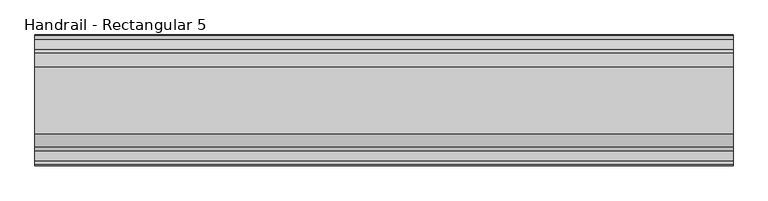
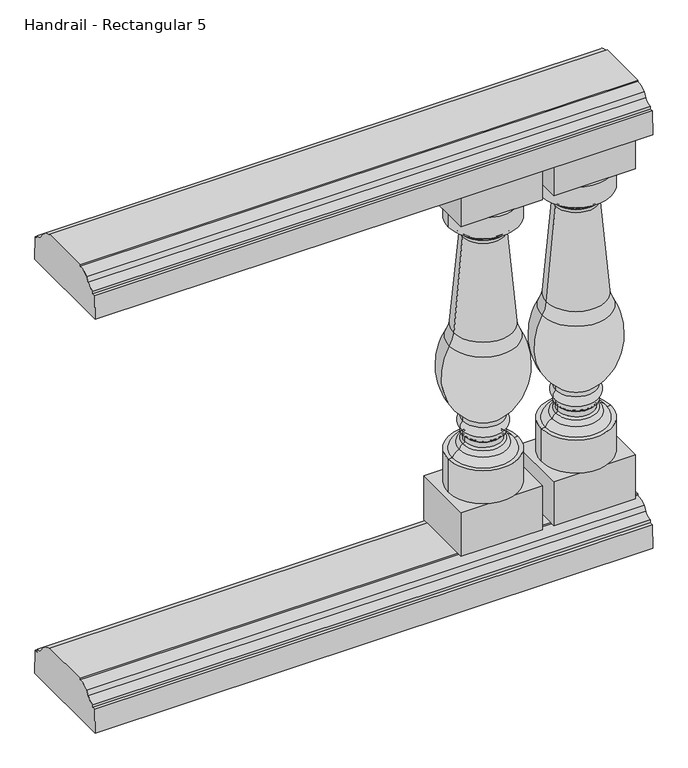
"""IFC4 building model written with IfcOpenShell, lengths in millimetres: railing geometry, Handrail - Rectangular 5."""

from ifc_helpers import new_model, si_unit, point, frame, frame_2d, origin, place, context, project, spatial, polyline, circle_curve, ellipse_curve, trimmed, segment, composite_curve, outline, extrude, source, transform, mapped, element, save
from ifc_brep_helpers import plane_surface, cylinder_surface, revolved_surface, advanced_brep


def handrail_rectangular_5_e4c3c7e0(model_context):
    return source(origin(), model_context, "Body", "SolidModel", [
        extrude(outline(composite_curve([segment(trimmed(circle_curve(frame_2d((-1771.1852268, 1054.89375)), 19.84375), [point((-1771.1852268, 1035.05))], [point((-1754.064785, 1044.8605607))], True, "CARTESIAN"), True, "CONTINUOUS"), segment(polyline([(-1754.064785, 1044.8605607), (-1747.604713, 1054.3201059)]), True, "CONTINUOUS"), segment(trimmed(circle_curve(frame_2d((-1723.5602268, 1027.90625)), 35.71875), [point((-1747.604713, 1054.3201059))], [point((-1723.5602268, 1063.625))], False, "CARTESIAN"), True, "CONTINUOUS"), segment(polyline([(-1723.5602268, 1063.625), (-1723.5602268, 1066.8), (-1607.6727268, 1066.8), (-1607.6727268, 1063.625)]), True, "CONTINUOUS"), segment(trimmed(circle_curve(frame_2d((-1607.6727268, 1027.90625)), 35.71875), [point((-1607.6727268, 1063.625))], [point((-1583.6282406, 1054.3201059))], False, "CARTESIAN"), True, "CONTINUOUS"), segment(polyline([(-1583.6282406, 1054.3201059), (-1577.1681686, 1044.8605607)]), True, "CONTINUOUS"), segment(trimmed(circle_curve(frame_2d((-1560.0477268, 1054.89375)), 19.84375), [point((-1577.1681686, 1044.8605607))], [point((-1560.0477268, 1035.05))], True, "CARTESIAN"), True, "CONTINUOUS"), segment(polyline([(-1560.0477268, 1035.05), (-1560.0477268, 1028.7), (-1552.9039768, 1028.7), (-1551.3164768, 974.725), (-1779.9164768, 974.725), (-1778.3289768, 1028.7), (-1771.1852268, 1028.7), (-1771.1852268, 1035.05)]), True, "CONTINUOUS")], self_intersect=False)), frame((16266.0521895, 0.0, 0.0), z_axis=(1.0, 0.0, 0.0), x_axis=(0.0, 1.0, 0.0)), (0.0, 0.0, 1.0), 1219.2),
        extrude(outline(composite_curve([segment(trimmed(circle_curve(frame_2d((-1771.1852268, 99.21875)), 19.84375), [point((-1771.1852268, 79.375))], [point((-1754.064785, 89.1855607))], True, "CARTESIAN"), True, "CONTINUOUS"), segment(polyline([(-1754.064785, 89.1855607), (-1747.604713, 98.6451059)]), True, "CONTINUOUS"), segment(trimmed(circle_curve(frame_2d((-1723.5602268, 72.23125)), 35.71875), [point((-1747.604713, 98.6451059))], [point((-1723.5602268, 107.95))], False, "CARTESIAN"), True, "CONTINUOUS"), segment(polyline([(-1723.5602268, 107.95), (-1723.5602268, 111.125), (-1607.6727268, 111.125), (-1607.6727268, 107.95)]), True, "CONTINUOUS"), segment(trimmed(circle_curve(frame_2d((-1607.6727268, 72.23125)), 35.71875), [point((-1607.6727268, 107.95))], [point((-1583.6282406, 98.6451059))], False, "CARTESIAN"), True, "CONTINUOUS"), segment(polyline([(-1583.6282406, 98.6451059), (-1577.1681686, 89.1855607)]), True, "CONTINUOUS"), segment(trimmed(circle_curve(frame_2d((-1560.0477268, 99.21875)), 19.84375), [point((-1577.1681686, 89.1855607))], [point((-1560.0477268, 79.375))], True, "CARTESIAN"), True, "CONTINUOUS"), segment(polyline([(-1560.0477268, 79.375), (-1560.0477268, 73.025), (-1552.9039768, 73.025), (-1551.3164768, 19.05), (-1779.9164768, 19.05), (-1778.3289768, 73.025), (-1771.1852268, 73.025), (-1771.1852268, 79.375)]), True, "CONTINUOUS")], self_intersect=False)), frame((16266.0521895, 0.0, 0.0), z_axis=(1.0, 0.0, 0.0), x_axis=(0.0, 1.0, 0.0)), (0.0, 0.0, 1.0), 1219.2),
        advanced_brep(
        [(17307.4521895, -1665.6164768, 873.125), (17459.8521895, -1665.6164768, 873.125), (17383.6521895, -1665.6164768, 873.125), (17307.4521895, -1665.6164768, 825.4490755), (17459.8521895, -1665.6164768, 825.4490755), (17317.4954208, -1665.6164768, 825.4490755), (17449.8089583, -1665.6164768, 825.4490755), (17328.9787107, -1665.6164768, 813.9657856), (17438.3256684, -1665.6164768, 813.9657856), (17328.9787107, -1665.6164768, 808.3461292), (17438.3256684, -1665.6164768, 808.3461292), (17334.6808978, -1665.6164768, 802.2016975), (17432.6234813, -1665.6164768, 802.2016975), (17338.0226936, -1665.6164768, 792.8428746), (17429.2816855, -1665.6164768, 792.8428746), (17319.2551876, -1665.6164768, 577.4758218), (17448.0491915, -1665.6164768, 577.4758218), (17310.237965, -1665.6164768, 549.5125844), (17457.0664141, -1665.6164768, 549.5125844), (17339.5087972, -1665.6164768, 376.7693301), (17427.7955818, -1665.6164768, 376.7693301), (17339.5087972, -1665.6164768, 366.4437154), (17427.7955818, -1665.6164768, 366.4437154), (17339.5087972, -1665.6164768, 343.8682651), (17427.7955818, -1665.6164768, 343.8682651), (17339.5087972, -1665.6164768, 333.5426504), (17427.7955818, -1665.6164768, 333.5426504), (17343.8192375, -1665.6164768, 329.2322102), (17423.4851416, -1665.6164768, 329.2322102), (17343.8192375, -1665.6164768, 317.4353211), (17423.4851416, -1665.6164768, 317.4353211), (17339.3214444, -1665.6164768, 313.1289544), (17427.9829347, -1665.6164768, 313.1289544), (17331.8009874, -1665.6164768, 303.0807869), (17435.5033917, -1665.6164768, 303.0807869), (17316.6523786, -1665.6164768, 288.925), (17450.6520004, -1665.6164768, 288.925), (17307.4521895, -1665.6164768, 288.925), (17459.8521895, -1665.6164768, 288.925), (17307.4521895, -1665.6164768, 212.725), (17459.8521895, -1665.6164768, 212.725), (17383.6521895, -1665.6164768, 212.725)],
        [
            (0, 1, circle_curve(frame((17383.6521895, -1665.6164768, 873.125), z_axis=(0.0, 0.0, 1.0), x_axis=(1.0, 0.0, 0.0)), 76.2)),
            (1, 2),
            (2, 0),
            (1, 0, circle_curve(frame((17383.6521895, -1665.6164768, 873.125), z_axis=(0.0, 0.0, 1.0), x_axis=(1.0, 0.0, 0.0)), 76.2)),
            (3, 4, circle_curve(frame((17383.6521895, -1665.6164768, 825.4490755), z_axis=(0.0, 0.0, 1.0), x_axis=(1.0, 0.0, 0.0)), 76.2)),
            (4, 1),
            (0, 3),
            (4, 3, circle_curve(frame((17383.6521895, -1665.6164768, 825.4490755), z_axis=(0.0, 0.0, 1.0), x_axis=(1.0, 0.0, 0.0)), 76.2)),
            (5, 6, circle_curve(frame((17383.6521895, -1665.6164768, 825.4490755), z_axis=(0.0, 0.0, 1.0), x_axis=(1.0, 0.0, 0.0)), 66.1567687)),
            (6, 4),
            (3, 5),
            (6, 5, circle_curve(frame((17383.6521895, -1665.6164768, 825.4490755), z_axis=(0.0, 0.0, 1.0), x_axis=(1.0, 0.0, 0.0)), 66.1567687)),
            (7, 8, circle_curve(frame((17383.6521895, -1665.6164768, 813.9657856), z_axis=(0.0, 0.0, 1.0), x_axis=(1.0, 0.0, 0.0)), 54.6734788)),
            (8, 6, circle_curve(frame((17438.3256684, -1665.6164768, 825.4490755), z_axis=(0.0, -1.0, 0.0), x_axis=(-1.0, 0.0, 0.0)), 11.4832899)),
            (5, 7, circle_curve(frame((17328.9787107, -1665.6164768, 825.4490755), z_axis=(0.0, -1.0, 0.0), x_axis=(1.0, 0.0, 0.0)), 11.4832899)),
            (8, 7, circle_curve(frame((17383.6521895, -1665.6164768, 813.9657856), z_axis=(0.0, 0.0, 1.0), x_axis=(1.0, 0.0, 0.0)), 54.6734788)),
            (9, 10, circle_curve(frame((17383.6521895, -1665.6164768, 808.3461292), z_axis=(0.0, 0.0, 1.0), x_axis=(1.0, 0.0, 0.0)), 54.6734788)),
            (10, 8),
            (7, 9),
            (10, 9, circle_curve(frame((17383.6521895, -1665.6164768, 808.3461292), z_axis=(0.0, 0.0, 1.0), x_axis=(1.0, 0.0, 0.0)), 54.6734788)),
            (11, 12, circle_curve(frame((17383.6521895, -1665.6164768, 802.2016975), z_axis=(0.0, 0.0, 1.0), x_axis=(1.0, 0.0, 0.0)), 48.9712918)),
            (12, 10, circle_curve(frame((17446.0345288, -1665.6164768, 795.4740105), z_axis=(0.0, 1.0, 0.0), x_axis=(-1.0, 0.0, 0.0)), 15.0039317)),
            (9, 11, circle_curve(frame((17321.2698503, -1665.6164768, 795.4740105), z_axis=(0.0, 1.0, 0.0), x_axis=(1.0, 0.0, 0.0)), 15.0039317)),
            (12, 11, circle_curve(frame((17383.6521895, -1665.6164768, 802.2016975), z_axis=(0.0, 0.0, 1.0), x_axis=(1.0, 0.0, 0.0)), 48.9712918)),
            (13, 14, circle_curve(frame((17383.6521895, -1665.6164768, 792.8428746), z_axis=(0.0, 0.0, 1.0), x_axis=(1.0, 0.0, 0.0)), 45.629496)),
            (14, 12, circle_curve(frame((17441.9595739, -1665.6164768, 793.5919719), z_axis=(0.0, 1.0, 0.0), x_axis=(-1.0, 0.0, 0.0)), 12.7)),
            (11, 13, circle_curve(frame((17325.3448052, -1665.6164768, 793.5919719), z_axis=(0.0, 1.0, 0.0), x_axis=(1.0, 0.0, 0.0)), 12.7)),
            (14, 13, circle_curve(frame((17383.6521895, -1665.6164768, 792.8428746), z_axis=(0.0, 0.0, 1.0), x_axis=(1.0, 0.0, 0.0)), 45.629496)),
            (15, 16, circle_curve(frame((17383.6521895, -1665.6164768, 577.4758218), z_axis=(0.0, 0.0, 1.0), x_axis=(1.0, 0.0, 0.0)), 64.3970019)),
            (16, 14, circle_curve(frame((21296.7232099, -1665.6164768, 1021.358044), z_axis=(0.0, 1.0, 0.0), x_axis=(-1.0, 0.0, 0.0)), 3874.1867698)),
            (13, 15, circle_curve(frame((13470.5811691, -1665.6164768, 1021.358044), z_axis=(0.0, 1.0, 0.0), x_axis=(1.0, 0.0, 0.0)), 3874.1867698)),
            (16, 15, circle_curve(frame((17383.6521895, -1665.6164768, 577.4758218), z_axis=(0.0, 0.0, 1.0), x_axis=(1.0, 0.0, 0.0)), 64.3970019)),
            (17, 18, circle_curve(frame((17383.6521895, -1665.6164768, 549.5125844), z_axis=(0.0, 0.0, 1.0), x_axis=(1.0, 0.0, 0.0)), 73.4142246)),
            (18, 16, circle_curve(frame((17522.5688441, -1665.6164768, 586.070457), z_axis=(0.0, 1.0, 0.0), x_axis=(-1.0, 0.0, 0.0)), 75.0136413)),
            (15, 17, circle_curve(frame((17244.735535, -1665.6164768, 586.070457), z_axis=(0.0, 1.0, 0.0), x_axis=(1.0, 0.0, 0.0)), 75.0136413)),
            (18, 17, circle_curve(frame((17383.6521895, -1665.6164768, 549.5125844), z_axis=(0.0, 0.0, 1.0), x_axis=(1.0, 0.0, 0.0)), 73.4142246)),
            (19, 20, circle_curve(frame((17383.6521895, -1665.6164768, 376.7693301), z_axis=(0.0, 0.0, 1.0), x_axis=(1.0, 0.0, 0.0)), 44.1433923)),
            (20, 18, circle_curve(frame((17334.9440648, -1665.6164768, 481.3542994), z_axis=(0.0, -1.0, 0.0), x_axis=(-1.0, 0.0, 0.0)), 139.8549964)),
            (17, 19, circle_curve(frame((17432.3603143, -1665.6164768, 481.3542994), z_axis=(0.0, -1.0, 0.0), x_axis=(1.0, 0.0, 0.0)), 139.8549964)),
            (20, 19, circle_curve(frame((17383.6521895, -1665.6164768, 376.7693301), z_axis=(0.0, 0.0, 1.0), x_axis=(1.0, 0.0, 0.0)), 44.1433923)),
            (21, 22, circle_curve(frame((17383.6521895, -1665.6164768, 366.4437154), z_axis=(0.0, 0.0, 1.0), x_axis=(1.0, 0.0, 0.0)), 44.1433923)),
            (22, 20),
            (19, 21),
            (22, 21, circle_curve(frame((17383.6521895, -1665.6164768, 366.4437154), z_axis=(0.0, 0.0, 1.0), x_axis=(1.0, 0.0, 0.0)), 44.1433923)),
            (23, 24, circle_curve(frame((17383.6521895, -1665.6164768, 343.8682651), z_axis=(0.0, 0.0, 1.0), x_axis=(1.0, 0.0, 0.0)), 44.1433923)),
            (24, 22, circle_curve(frame((17419.503554, -1665.6164768, 355.1559903), z_axis=(0.0, -1.0, 0.0), x_axis=(-1.0, 0.0, 0.0)), 14.0060867)),
            (21, 23, circle_curve(frame((17347.8008251, -1665.6164768, 355.1559903), z_axis=(0.0, -1.0, 0.0), x_axis=(1.0, 0.0, 0.0)), 14.0060867)),
            (24, 23, circle_curve(frame((17383.6521895, -1665.6164768, 343.8682651), z_axis=(0.0, 0.0, 1.0), x_axis=(1.0, 0.0, 0.0)), 44.1433923)),
            (25, 26, circle_curve(frame((17383.6521895, -1665.6164768, 333.5426504), z_axis=(0.0, 0.0, 1.0), x_axis=(1.0, 0.0, 0.0)), 44.1433923)),
            (26, 24),
            (23, 25),
            (26, 25, circle_curve(frame((17383.6521895, -1665.6164768, 333.5426504), z_axis=(0.0, 0.0, 1.0), x_axis=(1.0, 0.0, 0.0)), 44.1433923)),
            (27, 28, circle_curve(frame((17383.6521895, -1665.6164768, 329.2322102), z_axis=(0.0, 0.0, 1.0), x_axis=(1.0, 0.0, 0.0)), 39.8329521)),
            (28, 26, circle_curve(frame((17427.7955818, -1665.6164768, 329.2322102), z_axis=(0.0, 1.0, 0.0), x_axis=(-1.0, 0.0, 0.0)), 4.3104402)),
            (25, 27, circle_curve(frame((17339.5087972, -1665.6164768, 329.2322102), z_axis=(0.0, 1.0, 0.0), x_axis=(1.0, 0.0, 0.0)), 4.3104402)),
            (28, 27, circle_curve(frame((17383.6521895, -1665.6164768, 329.2322102), z_axis=(0.0, 0.0, 1.0), x_axis=(1.0, 0.0, 0.0)), 39.8329521)),
            (29, 30, circle_curve(frame((17383.6521895, -1665.6164768, 317.4353211), z_axis=(0.0, 0.0, 1.0), x_axis=(1.0, 0.0, 0.0)), 39.8329521)),
            (30, 28),
            (27, 29),
            (30, 29, circle_curve(frame((17383.6521895, -1665.6164768, 317.4353211), z_axis=(0.0, 0.0, 1.0), x_axis=(1.0, 0.0, 0.0)), 39.8329521)),
            (31, 32, circle_curve(frame((17383.6521895, -1665.6164768, 313.1289544), z_axis=(0.0, 0.0, 1.0), x_axis=(1.0, 0.0, 0.0)), 44.3307451)),
            (32, 30, circle_curve(frame((17427.7955818, -1665.6164768, 317.4353211), z_axis=(0.0, 1.0, 0.0), x_axis=(-1.0, 0.0, 0.0)), 4.3104402)),
            (29, 31, circle_curve(frame((17339.5087972, -1665.6164768, 317.4353211), z_axis=(0.0, 1.0, 0.0), x_axis=(1.0, 0.0, 0.0)), 4.3104402)),
            (32, 31, circle_curve(frame((17383.6521895, -1665.6164768, 313.1289544), z_axis=(0.0, 0.0, 1.0), x_axis=(1.0, 0.0, 0.0)), 44.3307451)),
            (33, 34, circle_curve(frame((17383.6521895, -1665.6164768, 303.0807869), z_axis=(0.0, 0.0, 1.0), x_axis=(1.0, 0.0, 0.0)), 51.8512022)),
            (34, 32, circle_curve(frame((17420.8640754, -1665.6164768, 299.962519), z_axis=(0.0, -1.0, 0.0), x_axis=(-1.0, 0.0, 0.0)), 14.9677378)),
            (31, 33, circle_curve(frame((17346.4403037, -1665.6164768, 299.962519), z_axis=(0.0, -1.0, 0.0), x_axis=(1.0, 0.0, 0.0)), 14.9677378)),
            (34, 33, circle_curve(frame((17383.6521895, -1665.6164768, 303.0807869), z_axis=(0.0, 0.0, 1.0), x_axis=(1.0, 0.0, 0.0)), 51.8512022)),
            (35, 36, circle_curve(frame((17383.6521895, -1665.6164768, 288.925), z_axis=(0.0, 0.0, 1.0), x_axis=(1.0, 0.0, 0.0)), 66.9998109)),
            (36, 34, circle_curve(frame((17430.2545436, -1665.6164768, 282.2803841), z_axis=(0.0, -1.0, 0.0), x_axis=(-1.0, 0.0, 0.0)), 21.4524396)),
            (33, 35, circle_curve(frame((17337.0498354, -1665.6164768, 282.2803841), z_axis=(0.0, -1.0, 0.0), x_axis=(1.0, 0.0, 0.0)), 21.4524396)),
            (36, 35, circle_curve(frame((17383.6521895, -1665.6164768, 288.925), z_axis=(0.0, 0.0, 1.0), x_axis=(1.0, 0.0, 0.0)), 66.9998109)),
            (37, 38, circle_curve(frame((17383.6521895, -1665.6164768, 288.925), z_axis=(0.0, 0.0, 1.0), x_axis=(1.0, 0.0, 0.0)), 76.2)),
            (38, 36),
            (35, 37),
            (38, 37, circle_curve(frame((17383.6521895, -1665.6164768, 288.925), z_axis=(0.0, 0.0, 1.0), x_axis=(1.0, 0.0, 0.0)), 76.2)),
            (39, 40, circle_curve(frame((17383.6521895, -1665.6164768, 212.725), z_axis=(0.0, 0.0, 1.0), x_axis=(1.0, 0.0, 0.0)), 76.2)),
            (40, 38),
            (37, 39),
            (40, 39, circle_curve(frame((17383.6521895, -1665.6164768, 212.725), z_axis=(0.0, 0.0, 1.0), x_axis=(1.0, 0.0, 0.0)), 76.2)),
            (41, 40),
            (39, 41),
        ],
        [
            plane_surface(frame((17383.6521895, -1665.6164768, 873.125), z_axis=(0.0, 0.0, 1.0), x_axis=(1.0, 0.0, 0.0))),
            cylinder_surface(frame((17383.6521895, -1665.6164768, 841.375), z_axis=(0.0, 0.0, -1.0), x_axis=(1.0, 0.0, 0.0)), 76.2),
            plane_surface(frame((17383.6521895, -1665.6164768, 825.4490755), z_axis=(0.0, 0.0, -1.0), x_axis=(1.0, 0.0, 0.0))),
            revolved_surface(trimmed(ellipse_curve(frame((17438.3256684, -1665.6164768, 825.4490755), z_axis=(0.0, 1.0, 0.0), x_axis=(-1.0, 0.0, 0.0)), 11.4832899, 11.4832899), [point((17449.8089583, -1665.6164768, 825.4490755))], [point((17438.3256684, -1665.6164768, 813.9657856))], True, "CARTESIAN"), (17383.6521895, -1665.6164768, 841.375), (0.0, 0.0, -1.0)),
            cylinder_surface(frame((17383.6521895, -1665.6164768, 841.375), z_axis=(0.0, 0.0, -1.0), x_axis=(1.0, 0.0, 0.0)), 54.6734788),
            revolved_surface(trimmed(ellipse_curve(frame((17446.0345288, -1665.6164768, 795.4740105), z_axis=(0.0, -1.0, 0.0), x_axis=(-1.0, 0.0, 0.0)), 15.0039317, 15.0039317), [point((17438.3256684, -1665.6164768, 808.3461292))], [point((17432.6234813, -1665.6164768, 802.2016975))], True, "CARTESIAN"), (17383.6521895, -1665.6164768, 841.375), (0.0, 0.0, -1.0)),
            revolved_surface(trimmed(ellipse_curve(frame((17441.9595739, -1665.6164768, 793.5919719), z_axis=(0.0, -1.0, 0.0), x_axis=(-1.0, 0.0, 0.0)), 12.7, 12.7), [point((17432.6234813, -1665.6164768, 802.2016975))], [point((17429.2816855, -1665.6164768, 792.8428746))], True, "CARTESIAN"), (17383.6521895, -1665.6164768, 841.375), (0.0, 0.0, -1.0)),
            revolved_surface(trimmed(ellipse_curve(frame((21296.7232099, -1665.6164768, 1021.358044), z_axis=(0.0, -1.0, 0.0), x_axis=(-1.0, 0.0, 0.0)), 3874.1867698, 3874.1867698), [point((17429.2816855, -1665.6164768, 792.8428746))], [point((17448.0491915, -1665.6164768, 577.4758218))], True, "CARTESIAN"), (17383.6521895, -1665.6164768, 841.375), (0.0, 0.0, -1.0)),
            revolved_surface(trimmed(ellipse_curve(frame((17522.5688441, -1665.6164768, 586.070457), z_axis=(0.0, -1.0, 0.0), x_axis=(-1.0, 0.0, 0.0)), 75.0136413, 75.0136413), [point((17448.0491915, -1665.6164768, 577.4758218))], [point((17457.0664141, -1665.6164768, 549.5125844))], True, "CARTESIAN"), (17383.6521895, -1665.6164768, 841.375), (0.0, 0.0, -1.0)),
            revolved_surface(trimmed(ellipse_curve(frame((17334.9440648, -1665.6164768, 481.3542994), z_axis=(0.0, 1.0, 0.0), x_axis=(-1.0, 0.0, 0.0)), 139.8549964, 139.8549964), [point((17457.0664141, -1665.6164768, 549.5125844))], [point((17427.7955818, -1665.6164768, 376.7693301))], True, "CARTESIAN"), (17383.6521895, -1665.6164768, 841.375), (0.0, 0.0, -1.0)),
            cylinder_surface(frame((17383.6521895, -1665.6164768, 841.375), z_axis=(0.0, 0.0, -1.0), x_axis=(1.0, 0.0, 0.0)), 44.1433923),
            revolved_surface(trimmed(ellipse_curve(frame((17419.503554, -1665.6164768, 355.1559903), z_axis=(0.0, 1.0, 0.0), x_axis=(-1.0, 0.0, 0.0)), 14.0060867, 14.0060867), [point((17427.7955818, -1665.6164768, 366.4437154))], [point((17427.7955818, -1665.6164768, 343.8682651))], True, "CARTESIAN"), (17383.6521895, -1665.6164768, 841.375), (0.0, 0.0, -1.0)),
            revolved_surface(trimmed(ellipse_curve(frame((17427.7955818, -1665.6164768, 329.2322102), z_axis=(0.0, -1.0, 0.0), x_axis=(-1.0, 0.0, 0.0)), 4.3104402, 4.3104402), [point((17427.7955818, -1665.6164768, 333.5426504))], [point((17423.4851416, -1665.6164768, 329.2322102))], True, "CARTESIAN"), (17383.6521895, -1665.6164768, 841.375), (0.0, 0.0, -1.0)),
            cylinder_surface(frame((17383.6521895, -1665.6164768, 841.375), z_axis=(0.0, 0.0, -1.0), x_axis=(1.0, 0.0, 0.0)), 39.8329521),
            revolved_surface(trimmed(ellipse_curve(frame((17427.7955818, -1665.6164768, 317.4353211), z_axis=(0.0, -1.0, 0.0), x_axis=(-1.0, 0.0, 0.0)), 4.3104402, 4.3104402), [point((17423.4851416, -1665.6164768, 317.4353211))], [point((17427.9829347, -1665.6164768, 313.1289544))], True, "CARTESIAN"), (17383.6521895, -1665.6164768, 841.375), (0.0, 0.0, -1.0)),
            revolved_surface(trimmed(ellipse_curve(frame((17420.8640754, -1665.6164768, 299.962519), z_axis=(0.0, 1.0, 0.0), x_axis=(-1.0, 0.0, 0.0)), 14.9677378, 14.9677378), [point((17427.9829347, -1665.6164768, 313.1289544))], [point((17435.5033917, -1665.6164768, 303.0807869))], True, "CARTESIAN"), (17383.6521895, -1665.6164768, 841.375), (0.0, 0.0, -1.0)),
            revolved_surface(trimmed(ellipse_curve(frame((17430.2545436, -1665.6164768, 282.2803841), z_axis=(0.0, 1.0, 0.0), x_axis=(-1.0, 0.0, 0.0)), 21.4524396, 21.4524396), [point((17435.5033917, -1665.6164768, 303.0807869))], [point((17450.6520004, -1665.6164768, 288.925))], True, "CARTESIAN"), (17383.6521895, -1665.6164768, 841.375), (0.0, 0.0, -1.0)),
            plane_surface(frame((17383.6521895, -1665.6164768, 288.925), z_axis=(0.0, 0.0, 1.0), x_axis=(1.0, 0.0, 0.0))),
            plane_surface(frame((17383.6521895, -1665.6164768, 212.725), z_axis=(0.0, 0.0, -1.0), x_axis=(1.0, 0.0, 0.0))),
        ],
        [
            (0, [[1, 2, 3]]),
            (0, [[4, -3, -2]]),
            (1, [[5, 6, -1, 7]]),
            (1, [[8, -7, -4, -6]]),
            (2, [[9, 10, -5, 11]]),
            (2, [[12, -11, -8, -10]]),
            (3, [[13, 14, -9, 15]]),
            (3, [[16, -15, -12, -14]]),
            (4, [[17, 18, -13, 19]]),
            (4, [[20, -19, -16, -18]]),
            (5, [[21, 22, -17, 23]]),
            (5, [[24, -23, -20, -22]]),
            (6, [[25, 26, -21, 27]]),
            (6, [[28, -27, -24, -26]]),
            (7, [[29, 30, -25, 31]]),
            (7, [[32, -31, -28, -30]]),
            (8, [[33, 34, -29, 35]]),
            (8, [[36, -35, -32, -34]]),
            (9, [[37, 38, -33, 39]]),
            (9, [[40, -39, -36, -38]]),
            (10, [[41, 42, -37, 43]]),
            (10, [[44, -43, -40, -42]]),
            (11, [[45, 46, -41, 47]]),
            (11, [[48, -47, -44, -46]]),
            (10, [[49, 50, -45, 51]]),
            (10, [[52, -51, -48, -50]]),
            (12, [[53, 54, -49, 55]]),
            (12, [[56, -55, -52, -54]]),
            (13, [[57, 58, -53, 59]]),
            (13, [[60, -59, -56, -58]]),
            (14, [[61, 62, -57, 63]]),
            (14, [[64, -63, -60, -62]]),
            (15, [[65, 66, -61, 67]]),
            (15, [[68, -67, -64, -66]]),
            (16, [[69, 70, -65, 71]]),
            (16, [[72, -71, -68, -70]]),
            (17, [[73, 74, -69, 75]]),
            (17, [[76, -75, -72, -74]]),
            (1, [[77, 78, -73, 79]]),
            (1, [[80, -79, -76, -78]]),
            (18, [[81, -77, 82]]),
            (18, [[-82, -80, -81]]),
        ],
    ),
        extrude(outline(polyline([(17294.7521895, -1735.4664768), (17294.7521895, -1595.7664768), (17472.5521895, -1595.7664768), (17472.5521895, -1735.4664768), (17294.7521895, -1735.4664768)])), frame((0.0, 0.0, 111.125), z_axis=(0.0, 0.0, 1.0), x_axis=(1.0, 0.0, 0.0)), (0.0, 0.0, 1.0), 101.6),
        extrude(outline(polyline([(17294.7521895, -1595.7664768), (17472.5521895, -1595.7664768), (17472.5521895, -1735.4664768), (17294.7521895, -1735.4664768), (17294.7521895, -1595.7664768)])), frame((0.0, 0.0, 873.125), z_axis=(0.0, 0.0, 1.0), x_axis=(1.0, 0.0, 0.0)), (0.0, 0.0, 1.0), 101.6),
        advanced_brep(
        [(17104.2521895, -1665.6164768, 873.125), (17256.6521895, -1665.6164768, 873.125), (17180.4521895, -1665.6164768, 873.125), (17104.2521895, -1665.6164768, 825.4490755), (17256.6521895, -1665.6164768, 825.4490755), (17114.2954208, -1665.6164768, 825.4490755), (17246.6089583, -1665.6164768, 825.4490755), (17125.7787107, -1665.6164768, 813.9657856), (17235.1256684, -1665.6164768, 813.9657856), (17125.7787107, -1665.6164768, 808.3461292), (17235.1256684, -1665.6164768, 808.3461292), (17131.4808978, -1665.6164768, 802.2016975), (17229.4234813, -1665.6164768, 802.2016975), (17134.8226936, -1665.6164768, 792.8428746), (17226.0816855, -1665.6164768, 792.8428746), (17116.0551876, -1665.6164768, 577.4758218), (17244.8491915, -1665.6164768, 577.4758218), (17107.037965, -1665.6164768, 549.5125844), (17253.8664141, -1665.6164768, 549.5125844), (17136.3087972, -1665.6164768, 376.7693301), (17224.5955818, -1665.6164768, 376.7693301), (17136.3087972, -1665.6164768, 366.4437154), (17224.5955818, -1665.6164768, 366.4437154), (17136.3087972, -1665.6164768, 343.8682651), (17224.5955818, -1665.6164768, 343.8682651), (17136.3087972, -1665.6164768, 333.5426504), (17224.5955818, -1665.6164768, 333.5426504), (17140.6192375, -1665.6164768, 329.2322102), (17220.2851416, -1665.6164768, 329.2322102), (17140.6192375, -1665.6164768, 317.4353211), (17220.2851416, -1665.6164768, 317.4353211), (17136.1214444, -1665.6164768, 313.1289544), (17224.7829347, -1665.6164768, 313.1289544), (17128.6009874, -1665.6164768, 303.0807869), (17232.3033917, -1665.6164768, 303.0807869), (17113.4523786, -1665.6164768, 288.925), (17247.4520004, -1665.6164768, 288.925), (17104.2521895, -1665.6164768, 288.925), (17256.6521895, -1665.6164768, 288.925), (17104.2521895, -1665.6164768, 212.725), (17256.6521895, -1665.6164768, 212.725), (17180.4521895, -1665.6164768, 212.725)],
        [
            (0, 1, circle_curve(frame((17180.4521895, -1665.6164768, 873.125), z_axis=(0.0, 0.0, 1.0), x_axis=(1.0, 0.0, 0.0)), 76.2)),
            (1, 2),
            (2, 0),
            (1, 0, circle_curve(frame((17180.4521895, -1665.6164768, 873.125), z_axis=(0.0, 0.0, 1.0), x_axis=(1.0, 0.0, 0.0)), 76.2)),
            (3, 4, circle_curve(frame((17180.4521895, -1665.6164768, 825.4490755), z_axis=(0.0, 0.0, 1.0), x_axis=(1.0, 0.0, 0.0)), 76.2)),
            (4, 1),
            (0, 3),
            (4, 3, circle_curve(frame((17180.4521895, -1665.6164768, 825.4490755), z_axis=(0.0, 0.0, 1.0), x_axis=(1.0, 0.0, 0.0)), 76.2)),
            (5, 6, circle_curve(frame((17180.4521895, -1665.6164768, 825.4490755), z_axis=(0.0, 0.0, 1.0), x_axis=(1.0, 0.0, 0.0)), 66.1567687)),
            (6, 4),
            (3, 5),
            (6, 5, circle_curve(frame((17180.4521895, -1665.6164768, 825.4490755), z_axis=(0.0, 0.0, 1.0), x_axis=(1.0, 0.0, 0.0)), 66.1567687)),
            (7, 8, circle_curve(frame((17180.4521895, -1665.6164768, 813.9657856), z_axis=(0.0, 0.0, 1.0), x_axis=(1.0, 0.0, 0.0)), 54.6734788)),
            (8, 6, circle_curve(frame((17235.1256684, -1665.6164768, 825.4490755), z_axis=(0.0, -1.0, 0.0), x_axis=(-1.0, 0.0, 0.0)), 11.4832899)),
            (5, 7, circle_curve(frame((17125.7787107, -1665.6164768, 825.4490755), z_axis=(0.0, -1.0, 0.0), x_axis=(1.0, 0.0, 0.0)), 11.4832899)),
            (8, 7, circle_curve(frame((17180.4521895, -1665.6164768, 813.9657856), z_axis=(0.0, 0.0, 1.0), x_axis=(1.0, 0.0, 0.0)), 54.6734788)),
            (9, 10, circle_curve(frame((17180.4521895, -1665.6164768, 808.3461292), z_axis=(0.0, 0.0, 1.0), x_axis=(1.0, 0.0, 0.0)), 54.6734788)),
            (10, 8),
            (7, 9),
            (10, 9, circle_curve(frame((17180.4521895, -1665.6164768, 808.3461292), z_axis=(0.0, 0.0, 1.0), x_axis=(1.0, 0.0, 0.0)), 54.6734788)),
            (11, 12, circle_curve(frame((17180.4521895, -1665.6164768, 802.2016975), z_axis=(0.0, 0.0, 1.0), x_axis=(1.0, 0.0, 0.0)), 48.9712918)),
            (12, 10, circle_curve(frame((17242.8345288, -1665.6164768, 795.4740105), z_axis=(0.0, 1.0, 0.0), x_axis=(-1.0, 0.0, 0.0)), 15.0039317)),
            (9, 11, circle_curve(frame((17118.0698503, -1665.6164768, 795.4740105), z_axis=(0.0, 1.0, 0.0), x_axis=(1.0, 0.0, 0.0)), 15.0039317)),
            (12, 11, circle_curve(frame((17180.4521895, -1665.6164768, 802.2016975), z_axis=(0.0, 0.0, 1.0), x_axis=(1.0, 0.0, 0.0)), 48.9712918)),
            (13, 14, circle_curve(frame((17180.4521895, -1665.6164768, 792.8428746), z_axis=(0.0, 0.0, 1.0), x_axis=(1.0, 0.0, 0.0)), 45.629496)),
            (14, 12, circle_curve(frame((17238.7595739, -1665.6164768, 793.5919719), z_axis=(0.0, 1.0, 0.0), x_axis=(-1.0, 0.0, 0.0)), 12.7)),
            (11, 13, circle_curve(frame((17122.1448052, -1665.6164768, 793.5919719), z_axis=(0.0, 1.0, 0.0), x_axis=(1.0, 0.0, 0.0)), 12.7)),
            (14, 13, circle_curve(frame((17180.4521895, -1665.6164768, 792.8428746), z_axis=(0.0, 0.0, 1.0), x_axis=(1.0, 0.0, 0.0)), 45.629496)),
            (15, 16, circle_curve(frame((17180.4521895, -1665.6164768, 577.4758218), z_axis=(0.0, 0.0, 1.0), x_axis=(1.0, 0.0, 0.0)), 64.3970019)),
            (16, 14, circle_curve(frame((21093.5232099, -1665.6164768, 1021.358044), z_axis=(0.0, 1.0, 0.0), x_axis=(-1.0, 0.0, 0.0)), 3874.1867698)),
            (13, 15, circle_curve(frame((13267.3811691, -1665.6164768, 1021.358044), z_axis=(0.0, 1.0, 0.0), x_axis=(1.0, 0.0, 0.0)), 3874.1867698)),
            (16, 15, circle_curve(frame((17180.4521895, -1665.6164768, 577.4758218), z_axis=(0.0, 0.0, 1.0), x_axis=(1.0, 0.0, 0.0)), 64.3970019)),
            (17, 18, circle_curve(frame((17180.4521895, -1665.6164768, 549.5125844), z_axis=(0.0, 0.0, 1.0), x_axis=(1.0, 0.0, 0.0)), 73.4142246)),
            (18, 16, circle_curve(frame((17319.3688441, -1665.6164768, 586.070457), z_axis=(0.0, 1.0, 0.0), x_axis=(-1.0, 0.0, 0.0)), 75.0136413)),
            (15, 17, circle_curve(frame((17041.535535, -1665.6164768, 586.070457), z_axis=(0.0, 1.0, 0.0), x_axis=(1.0, 0.0, 0.0)), 75.0136413)),
            (18, 17, circle_curve(frame((17180.4521895, -1665.6164768, 549.5125844), z_axis=(0.0, 0.0, 1.0), x_axis=(1.0, 0.0, 0.0)), 73.4142246)),
            (19, 20, circle_curve(frame((17180.4521895, -1665.6164768, 376.7693301), z_axis=(0.0, 0.0, 1.0), x_axis=(1.0, 0.0, 0.0)), 44.1433923)),
            (20, 18, circle_curve(frame((17131.7440648, -1665.6164768, 481.3542994), z_axis=(0.0, -1.0, 0.0), x_axis=(-1.0, 0.0, 0.0)), 139.8549964)),
            (17, 19, circle_curve(frame((17229.1603143, -1665.6164768, 481.3542994), z_axis=(0.0, -1.0, 0.0), x_axis=(1.0, 0.0, 0.0)), 139.8549964)),
            (20, 19, circle_curve(frame((17180.4521895, -1665.6164768, 376.7693301), z_axis=(0.0, 0.0, 1.0), x_axis=(1.0, 0.0, 0.0)), 44.1433923)),
            (21, 22, circle_curve(frame((17180.4521895, -1665.6164768, 366.4437154), z_axis=(0.0, 0.0, 1.0), x_axis=(1.0, 0.0, 0.0)), 44.1433923)),
            (22, 20),
            (19, 21),
            (22, 21, circle_curve(frame((17180.4521895, -1665.6164768, 366.4437154), z_axis=(0.0, 0.0, 1.0), x_axis=(1.0, 0.0, 0.0)), 44.1433923)),
            (23, 24, circle_curve(frame((17180.4521895, -1665.6164768, 343.8682651), z_axis=(0.0, 0.0, 1.0), x_axis=(1.0, 0.0, 0.0)), 44.1433923)),
            (24, 22, circle_curve(frame((17216.303554, -1665.6164768, 355.1559903), z_axis=(0.0, -1.0, 0.0), x_axis=(-1.0, 0.0, 0.0)), 14.0060867)),
            (21, 23, circle_curve(frame((17144.6008251, -1665.6164768, 355.1559903), z_axis=(0.0, -1.0, 0.0), x_axis=(1.0, 0.0, 0.0)), 14.0060867)),
            (24, 23, circle_curve(frame((17180.4521895, -1665.6164768, 343.8682651), z_axis=(0.0, 0.0, 1.0), x_axis=(1.0, 0.0, 0.0)), 44.1433923)),
            (25, 26, circle_curve(frame((17180.4521895, -1665.6164768, 333.5426504), z_axis=(0.0, 0.0, 1.0), x_axis=(1.0, 0.0, 0.0)), 44.1433923)),
            (26, 24),
            (23, 25),
            (26, 25, circle_curve(frame((17180.4521895, -1665.6164768, 333.5426504), z_axis=(0.0, 0.0, 1.0), x_axis=(1.0, 0.0, 0.0)), 44.1433923)),
            (27, 28, circle_curve(frame((17180.4521895, -1665.6164768, 329.2322102), z_axis=(0.0, 0.0, 1.0), x_axis=(1.0, 0.0, 0.0)), 39.8329521)),
            (28, 26, circle_curve(frame((17224.5955818, -1665.6164768, 329.2322102), z_axis=(0.0, 1.0, 0.0), x_axis=(-1.0, 0.0, 0.0)), 4.3104402)),
            (25, 27, circle_curve(frame((17136.3087972, -1665.6164768, 329.2322102), z_axis=(0.0, 1.0, 0.0), x_axis=(1.0, 0.0, 0.0)), 4.3104402)),
            (28, 27, circle_curve(frame((17180.4521895, -1665.6164768, 329.2322102), z_axis=(0.0, 0.0, 1.0), x_axis=(1.0, 0.0, 0.0)), 39.8329521)),
            (29, 30, circle_curve(frame((17180.4521895, -1665.6164768, 317.4353211), z_axis=(0.0, 0.0, 1.0), x_axis=(1.0, 0.0, 0.0)), 39.8329521)),
            (30, 28),
            (27, 29),
            (30, 29, circle_curve(frame((17180.4521895, -1665.6164768, 317.4353211), z_axis=(0.0, 0.0, 1.0), x_axis=(1.0, 0.0, 0.0)), 39.8329521)),
            (31, 32, circle_curve(frame((17180.4521895, -1665.6164768, 313.1289544), z_axis=(0.0, 0.0, 1.0), x_axis=(1.0, 0.0, 0.0)), 44.3307451)),
            (32, 30, circle_curve(frame((17224.5955818, -1665.6164768, 317.4353211), z_axis=(0.0, 1.0, 0.0), x_axis=(-1.0, 0.0, 0.0)), 4.3104402)),
            (29, 31, circle_curve(frame((17136.3087972, -1665.6164768, 317.4353211), z_axis=(0.0, 1.0, 0.0), x_axis=(1.0, 0.0, 0.0)), 4.3104402)),
            (32, 31, circle_curve(frame((17180.4521895, -1665.6164768, 313.1289544), z_axis=(0.0, 0.0, 1.0), x_axis=(1.0, 0.0, 0.0)), 44.3307451)),
            (33, 34, circle_curve(frame((17180.4521895, -1665.6164768, 303.0807869), z_axis=(0.0, 0.0, 1.0), x_axis=(1.0, 0.0, 0.0)), 51.8512022)),
            (34, 32, circle_curve(frame((17217.6640754, -1665.6164768, 299.962519), z_axis=(0.0, -1.0, 0.0), x_axis=(-1.0, 0.0, 0.0)), 14.9677378)),
            (31, 33, circle_curve(frame((17143.2403037, -1665.6164768, 299.962519), z_axis=(0.0, -1.0, 0.0), x_axis=(1.0, 0.0, 0.0)), 14.9677378)),
            (34, 33, circle_curve(frame((17180.4521895, -1665.6164768, 303.0807869), z_axis=(0.0, 0.0, 1.0), x_axis=(1.0, 0.0, 0.0)), 51.8512022)),
            (35, 36, circle_curve(frame((17180.4521895, -1665.6164768, 288.925), z_axis=(0.0, 0.0, 1.0), x_axis=(1.0, 0.0, 0.0)), 66.9998109)),
            (36, 34, circle_curve(frame((17227.0545436, -1665.6164768, 282.2803841), z_axis=(0.0, -1.0, 0.0), x_axis=(-1.0, 0.0, 0.0)), 21.4524396)),
            (33, 35, circle_curve(frame((17133.8498354, -1665.6164768, 282.2803841), z_axis=(0.0, -1.0, 0.0), x_axis=(1.0, 0.0, 0.0)), 21.4524396)),
            (36, 35, circle_curve(frame((17180.4521895, -1665.6164768, 288.925), z_axis=(0.0, 0.0, 1.0), x_axis=(1.0, 0.0, 0.0)), 66.9998109)),
            (37, 38, circle_curve(frame((17180.4521895, -1665.6164768, 288.925), z_axis=(0.0, 0.0, 1.0), x_axis=(1.0, 0.0, 0.0)), 76.2)),
            (38, 36),
            (35, 37),
            (38, 37, circle_curve(frame((17180.4521895, -1665.6164768, 288.925), z_axis=(0.0, 0.0, 1.0), x_axis=(1.0, 0.0, 0.0)), 76.2)),
            (39, 40, circle_curve(frame((17180.4521895, -1665.6164768, 212.725), z_axis=(0.0, 0.0, 1.0), x_axis=(1.0, 0.0, 0.0)), 76.2)),
            (40, 38),
            (37, 39),
            (40, 39, circle_curve(frame((17180.4521895, -1665.6164768, 212.725), z_axis=(0.0, 0.0, 1.0), x_axis=(1.0, 0.0, 0.0)), 76.2)),
            (41, 40),
            (39, 41),
        ],
        [
            plane_surface(frame((17180.4521895, -1665.6164768, 873.125), z_axis=(0.0, 0.0, 1.0), x_axis=(1.0, 0.0, 0.0))),
            cylinder_surface(frame((17180.4521895, -1665.6164768, 841.375), z_axis=(0.0, 0.0, -1.0), x_axis=(1.0, 0.0, 0.0)), 76.2),
            plane_surface(frame((17180.4521895, -1665.6164768, 825.4490755), z_axis=(0.0, 0.0, -1.0), x_axis=(1.0, 0.0, 0.0))),
            revolved_surface(trimmed(ellipse_curve(frame((17235.1256684, -1665.6164768, 825.4490755), z_axis=(0.0, 1.0, 0.0), x_axis=(-1.0, 0.0, 0.0)), 11.4832899, 11.4832899), [point((17246.6089583, -1665.6164768, 825.4490755))], [point((17235.1256684, -1665.6164768, 813.9657856))], True, "CARTESIAN"), (17180.4521895, -1665.6164768, 841.375), (0.0, 0.0, -1.0)),
            cylinder_surface(frame((17180.4521895, -1665.6164768, 841.375), z_axis=(0.0, 0.0, -1.0), x_axis=(1.0, 0.0, 0.0)), 54.6734788),
            revolved_surface(trimmed(ellipse_curve(frame((17242.8345288, -1665.6164768, 795.4740105), z_axis=(0.0, -1.0, 0.0), x_axis=(-1.0, 0.0, 0.0)), 15.0039317, 15.0039317), [point((17235.1256684, -1665.6164768, 808.3461292))], [point((17229.4234813, -1665.6164768, 802.2016975))], True, "CARTESIAN"), (17180.4521895, -1665.6164768, 841.375), (0.0, 0.0, -1.0)),
            revolved_surface(trimmed(ellipse_curve(frame((17238.7595739, -1665.6164768, 793.5919719), z_axis=(0.0, -1.0, 0.0), x_axis=(-1.0, 0.0, 0.0)), 12.7, 12.7), [point((17229.4234813, -1665.6164768, 802.2016975))], [point((17226.0816855, -1665.6164768, 792.8428746))], True, "CARTESIAN"), (17180.4521895, -1665.6164768, 841.375), (0.0, 0.0, -1.0)),
            revolved_surface(trimmed(ellipse_curve(frame((21093.5232099, -1665.6164768, 1021.358044), z_axis=(0.0, -1.0, 0.0), x_axis=(-1.0, 0.0, 0.0)), 3874.1867698, 3874.1867698), [point((17226.0816855, -1665.6164768, 792.8428746))], [point((17244.8491915, -1665.6164768, 577.4758218))], True, "CARTESIAN"), (17180.4521895, -1665.6164768, 841.375), (0.0, 0.0, -1.0)),
            revolved_surface(trimmed(ellipse_curve(frame((17319.3688441, -1665.6164768, 586.070457), z_axis=(0.0, -1.0, 0.0), x_axis=(-1.0, 0.0, 0.0)), 75.0136413, 75.0136413), [point((17244.8491915, -1665.6164768, 577.4758218))], [point((17253.8664141, -1665.6164768, 549.5125844))], True, "CARTESIAN"), (17180.4521895, -1665.6164768, 841.375), (0.0, 0.0, -1.0)),
            revolved_surface(trimmed(ellipse_curve(frame((17131.7440648, -1665.6164768, 481.3542994), z_axis=(0.0, 1.0, 0.0), x_axis=(-1.0, 0.0, 0.0)), 139.8549964, 139.8549964), [point((17253.8664141, -1665.6164768, 549.5125844))], [point((17224.5955818, -1665.6164768, 376.7693301))], True, "CARTESIAN"), (17180.4521895, -1665.6164768, 841.375), (0.0, 0.0, -1.0)),
            cylinder_surface(frame((17180.4521895, -1665.6164768, 841.375), z_axis=(0.0, 0.0, -1.0), x_axis=(1.0, 0.0, 0.0)), 44.1433923),
            revolved_surface(trimmed(ellipse_curve(frame((17216.303554, -1665.6164768, 355.1559903), z_axis=(0.0, 1.0, 0.0), x_axis=(-1.0, 0.0, 0.0)), 14.0060867, 14.0060867), [point((17224.5955818, -1665.6164768, 366.4437154))], [point((17224.5955818, -1665.6164768, 343.8682651))], True, "CARTESIAN"), (17180.4521895, -1665.6164768, 841.375), (0.0, 0.0, -1.0)),
            revolved_surface(trimmed(ellipse_curve(frame((17224.5955818, -1665.6164768, 329.2322102), z_axis=(0.0, -1.0, 0.0), x_axis=(-1.0, 0.0, 0.0)), 4.3104402, 4.3104402), [point((17224.5955818, -1665.6164768, 333.5426504))], [point((17220.2851416, -1665.6164768, 329.2322102))], True, "CARTESIAN"), (17180.4521895, -1665.6164768, 841.375), (0.0, 0.0, -1.0)),
            cylinder_surface(frame((17180.4521895, -1665.6164768, 841.375), z_axis=(0.0, 0.0, -1.0), x_axis=(1.0, 0.0, 0.0)), 39.8329521),
            revolved_surface(trimmed(ellipse_curve(frame((17224.5955818, -1665.6164768, 317.4353211), z_axis=(0.0, -1.0, 0.0), x_axis=(-1.0, 0.0, 0.0)), 4.3104402, 4.3104402), [point((17220.2851416, -1665.6164768, 317.4353211))], [point((17224.7829347, -1665.6164768, 313.1289544))], True, "CARTESIAN"), (17180.4521895, -1665.6164768, 841.375), (0.0, 0.0, -1.0)),
            revolved_surface(trimmed(ellipse_curve(frame((17217.6640754, -1665.6164768, 299.962519), z_axis=(0.0, 1.0, 0.0), x_axis=(-1.0, 0.0, 0.0)), 14.9677378, 14.9677378), [point((17224.7829347, -1665.6164768, 313.1289544))], [point((17232.3033917, -1665.6164768, 303.0807869))], True, "CARTESIAN"), (17180.4521895, -1665.6164768, 841.375), (0.0, 0.0, -1.0)),
            revolved_surface(trimmed(ellipse_curve(frame((17227.0545436, -1665.6164768, 282.2803841), z_axis=(0.0, 1.0, 0.0), x_axis=(-1.0, 0.0, 0.0)), 21.4524396, 21.4524396), [point((17232.3033917, -1665.6164768, 303.0807869))], [point((17247.4520004, -1665.6164768, 288.925))], True, "CARTESIAN"), (17180.4521895, -1665.6164768, 841.375), (0.0, 0.0, -1.0)),
            plane_surface(frame((17180.4521895, -1665.6164768, 288.925), z_axis=(0.0, 0.0, 1.0), x_axis=(1.0, 0.0, 0.0))),
            plane_surface(frame((17180.4521895, -1665.6164768, 212.725), z_axis=(0.0, 0.0, -1.0), x_axis=(1.0, 0.0, 0.0))),
        ],
        [
            (0, [[1, 2, 3]]),
            (0, [[4, -3, -2]]),
            (1, [[5, 6, -1, 7]]),
            (1, [[8, -7, -4, -6]]),
            (2, [[9, 10, -5, 11]]),
            (2, [[12, -11, -8, -10]]),
            (3, [[13, 14, -9, 15]]),
            (3, [[16, -15, -12, -14]]),
            (4, [[17, 18, -13, 19]]),
            (4, [[20, -19, -16, -18]]),
            (5, [[21, 22, -17, 23]]),
            (5, [[24, -23, -20, -22]]),
            (6, [[25, 26, -21, 27]]),
            (6, [[28, -27, -24, -26]]),
            (7, [[29, 30, -25, 31]]),
            (7, [[32, -31, -28, -30]]),
            (8, [[33, 34, -29, 35]]),
            (8, [[36, -35, -32, -34]]),
            (9, [[37, 38, -33, 39]]),
            (9, [[40, -39, -36, -38]]),
            (10, [[41, 42, -37, 43]]),
            (10, [[44, -43, -40, -42]]),
            (11, [[45, 46, -41, 47]]),
            (11, [[48, -47, -44, -46]]),
            (10, [[49, 50, -45, 51]]),
            (10, [[52, -51, -48, -50]]),
            (12, [[53, 54, -49, 55]]),
            (12, [[56, -55, -52, -54]]),
            (13, [[57, 58, -53, 59]]),
            (13, [[60, -59, -56, -58]]),
            (14, [[61, 62, -57, 63]]),
            (14, [[64, -63, -60, -62]]),
            (15, [[65, 66, -61, 67]]),
            (15, [[68, -67, -64, -66]]),
            (16, [[69, 70, -65, 71]]),
            (16, [[72, -71, -68, -70]]),
            (17, [[73, 74, -69, 75]]),
            (17, [[76, -75, -72, -74]]),
            (1, [[77, 78, -73, 79]]),
            (1, [[80, -79, -76, -78]]),
            (18, [[81, -77, 82]]),
            (18, [[-82, -80, -81]]),
        ],
    ),
        extrude(outline(polyline([(17091.5521895, -1735.4664768), (17091.5521895, -1595.7664768), (17269.3521895, -1595.7664768), (17269.3521895, -1735.4664768), (17091.5521895, -1735.4664768)])), frame((0.0, 0.0, 111.125), z_axis=(0.0, 0.0, 1.0), x_axis=(1.0, 0.0, 0.0)), (0.0, 0.0, 1.0), 101.6),
        extrude(outline(polyline([(17091.5521895, -1595.7664768), (17269.3521895, -1595.7664768), (17269.3521895, -1735.4664768), (17091.5521895, -1735.4664768), (17091.5521895, -1595.7664768)])), frame((0.0, 0.0, 873.125), z_axis=(0.0, 0.0, 1.0), x_axis=(1.0, 0.0, 0.0)), (0.0, 0.0, 1.0), 101.6),
    ])


if __name__ == "__main__":
    model = new_model("IFC4")
    model_context = context("Model", 3, world=origin())
    ifc_project = project(units=[si_unit("LENGTHUNIT", "METRE", prefix="MILLI")], contexts=[model_context])
    site = spatial("IfcSite", under=ifc_project)
    building = spatial("IfcBuilding", under=site)
    placement = place(None, origin())
    handrail_rectangular_5_shape = handrail_rectangular_5_e4c3c7e0(model_context)
    element("IfcRailing", 1, ObjectType="Handrail - Rectangular 5", at=placement, inside=building, context=model_context, shape_type="MappedRepresentation", body=[
        mapped(handrail_rectangular_5_shape, transform((0.0, 0.0, 0.0), x_axis=(1.0, 0.0, 0.0), y_axis=(0.0, 1.0, 0.0), z_axis=(0.0, 0.0, 1.0))),
    ])
    save(model, "model.ifc")
